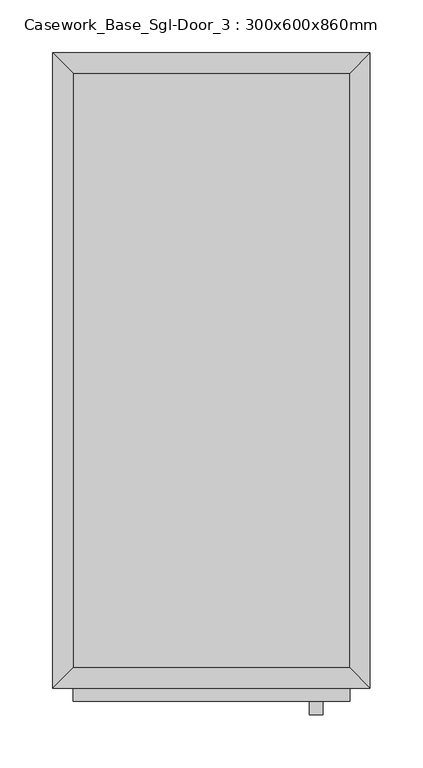
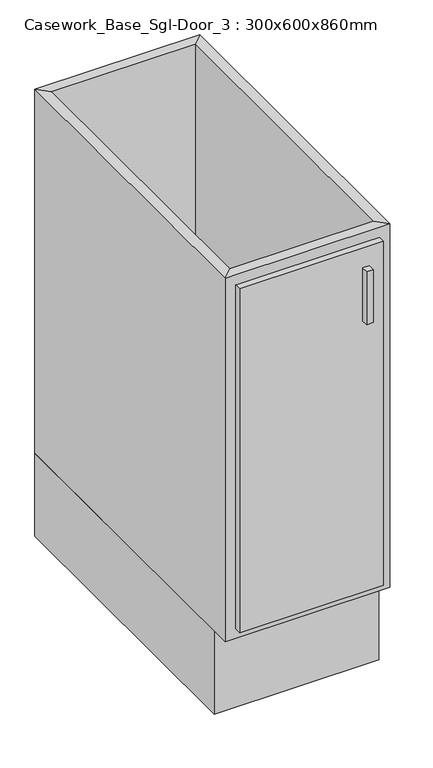
"""IFC4 building model written with IfcOpenShell, lengths in millimetres: furniture geometry, Casework_Base_Sgl-Door_3 : 300x600x860mm."""

import ifcopenshell
import ifcopenshell.guid

model = None  # the IFC model being written
_history = None  # IfcOwnerHistory: only IFC2X3 demands one
_inside = {}  # id of a spatial element -> (the spatial element, [elements in it])
_under = {}  # id of a project, library or spatial element -> (it, [spatial elements below it])
_declared = {}  # id of a project -> (the project, [libraries it declares])
_typed = {}  # id of a type object -> (the type object, [elements of that type])
_made_of = {}  # id of a material, layer set ... -> (it, [elements and type objects made of it])


def new_model(schema):
    """Start an empty IFC model of exactly this schema.

    Asked for "IFC4X3", IfcOpenShell would pick the latest addendum, in which some entities
    have other attributes; the version numbers below select the first issue.
    IFC2X3 requires an IfcOwnerHistory on every rooted entity: one is made here for all.
    """
    global model, _history
    if schema == "IFC4X3":
        model = ifcopenshell.file(schema_version=(4, 3, 0, 0))
    else:
        model = ifcopenshell.file(schema=schema)
    _inside.clear()
    _under.clear()
    _declared.clear()
    _typed.clear()
    _made_of.clear()
    _history = None
    if model.schema == "IFC2X3":
        org = make("IfcOrganization", Name="unknown")
        user = make(
            "IfcPersonAndOrganization",
            ThePerson=make("IfcPerson", FamilyName="unknown"),
            TheOrganization=org,
        )
        app = make(
            "IfcApplication",
            ApplicationDeveloper=org,
            Version="unknown",
            ApplicationFullName="unknown",
            ApplicationIdentifier="unknown",
        )
        _history = make(
            "IfcOwnerHistory",
            OwningUser=user,
            OwningApplication=app,
            ChangeAction="ADDED",
            CreationDate=0,
        )
    return model


def make(cls, **values):
    """One entity of the class cls with the attributes given. An attribute that is None is left unset."""
    return model.create_entity(
        cls, **{name: value for name, value in values.items() if value is not None}
    )


def rooted(cls, **values):
    """An entity with a GlobalId (a new one), such as an element, a storey or a relation."""
    return make(cls, GlobalId=ifcopenshell.guid.new(), OwnerHistory=_history, **values)


def si_unit(unit_type, name, prefix=None):
    """IfcSIUnit, for example si_unit("LENGTHUNIT", "METRE", prefix="MILLI")."""
    return make("IfcSIUnit", UnitType=unit_type, Prefix=prefix, Name=name)


def assignment(units):
    """IfcUnitAssignment: the units of a project."""
    return None if units is None else make("IfcUnitAssignment", Units=units)


def point(xyz):
    """IfcCartesianPoint."""
    return None if xyz is None else make("IfcCartesianPoint", Coordinates=xyz)


def direction(xyz):
    """IfcDirection."""
    return None if xyz is None else make("IfcDirection", DirectionRatios=xyz)


def frame(location, z_axis=None, x_axis=None):
    """IfcAxis2Placement3D, a coordinate frame: its origin and axes. An axis left out is left unset."""
    return make(
        "IfcAxis2Placement3D",
        Location=point(location),
        Axis=direction(z_axis),
        RefDirection=direction(x_axis),
    )


def origin():
    """The frame at (0, 0, 0) with its axes left unset."""
    return frame((0.0, 0.0, 0.0))


def origin_with_axes():
    """The frame at (0, 0, 0) with the z axis (0, 0, 1) and the x axis (1, 0, 0) written out."""
    return frame((0.0, 0.0, 0.0), z_axis=(0.0, 0.0, 1.0), x_axis=(1.0, 0.0, 0.0))


def place(relative_to, where):
    """IfcLocalPlacement: puts the frame where relative to a parent placement (None: the world)."""
    return make(
        "IfcLocalPlacement", PlacementRelTo=relative_to, RelativePlacement=where
    )


def context(
    kind, dimensions, precision=None, world=None, true_north=None, identifier=None
):
    """IfcGeometricRepresentationContext, for example the 3D "Model" context."""
    return make(
        "IfcGeometricRepresentationContext",
        ContextIdentifier=identifier,
        ContextType=kind,
        CoordinateSpaceDimension=dimensions,
        Precision=precision,
        WorldCoordinateSystem=world,
        TrueNorth=true_north,
    )


def project(units=None, contexts=None):
    """IfcProject with its units and contexts."""
    return rooted(
        "IfcProject",
        Name="project",
        RepresentationContexts=contexts,
        UnitsInContext=assignment(units),
    )


def spatial(cls, under=None, at=None, **own):
    """A site, building, storey or space (cls), placed at a placement, below another one or the project."""
    s = rooted(cls, ObjectPlacement=at, **own)
    if under is not None:
        _under.setdefault(under.id(), (under, []))[1].append(s)
    return s


def polyline(points):
    """IfcPolyline through the points."""
    return make("IfcPolyline", Points=[point(p) for p in points])


def outline(outer, holes=None, kind="AREA"):
    """IfcArbitraryClosedProfileDef: a profile drawn as a closed curve; with holes, ...WithVoids."""
    if holes is None:
        return make("IfcArbitraryClosedProfileDef", ProfileType=kind, OuterCurve=outer)
    return make(
        "IfcArbitraryProfileDefWithVoids",
        ProfileType=kind,
        OuterCurve=outer,
        InnerCurves=holes,
    )


def extrude(swept, where, along, depth):
    """IfcExtrudedAreaSolid: the profile swept, set in the frame where, extruded along a direction by depth."""
    return make(
        "IfcExtrudedAreaSolid",
        SweptArea=swept,
        Position=where,
        ExtrudedDirection=direction(along),
        Depth=depth,
    )


def faces_of(points, faces, orient=None, outer=None):
    """IfcFace entities. A face is a list of loops; a loop is a list of indices into points, from 0.

    orient and outer hold one flag for each loop. By default every Orientation is true, the
    first loop of a face is its IfcFaceOuterBound and the others are IfcFaceBound.
    """
    made = []
    for i, loops in enumerate(faces):
        bounds = []
        for j, loop in enumerate(loops):
            is_outer = j == 0 if outer is None else outer[i][j]
            bounds.append(
                make(
                    "IfcFaceOuterBound" if is_outer else "IfcFaceBound",
                    Bound=make("IfcPolyLoop", Polygon=[points[k] for k in loop]),
                    Orientation=True if orient is None else orient[i][j],
                )
            )
        made.append(make("IfcFace", Bounds=bounds))
    return made


def faceted_brep(points, faces, orient=None, outer=None, voids=None):
    """IfcFacetedBrep: a solid bounded by flat faces; with voids (closed shells), ...WithVoids."""
    shared = [point(p) for p in points]
    hull = make("IfcClosedShell", CfsFaces=faces_of(shared, faces, orient, outer))
    if voids is None:
        return make("IfcFacetedBrep", Outer=hull)
    return make(
        "IfcFacetedBrepWithVoids",
        Outer=hull,
        Voids=[
            make(cls, CfsFaces=faces_of(shared, fs, o, b)) for cls, fs, o, b in voids
        ],
    )


def shape(context_of_items, identifier, shape_type, items):
    """IfcShapeRepresentation: the items that make up one representation, for example the "Body"."""
    return make(
        "IfcShapeRepresentation",
        ContextOfItems=context_of_items,
        RepresentationIdentifier=identifier,
        RepresentationType=shape_type,
        Items=items,
    )


def source(mapping_origin, context_of_items, identifier, shape_type, items):
    """IfcRepresentationMap: a shape defined once, which mapped items show again and again."""
    return make(
        "IfcRepresentationMap",
        MappingOrigin=mapping_origin,
        MappedRepresentation=shape(context_of_items, identifier, shape_type, items),
    )


def transform(
    local_origin,
    x_axis=None,
    y_axis=None,
    z_axis=None,
    scale=None,
    scale2=None,
    scale3=None,
    uniform=True,
):
    """IfcCartesianTransformationOperator3D, or its non-uniform kind. x_axis, y_axis, z_axis: its Axis1, 2, 3."""
    if uniform:
        return make(
            "IfcCartesianTransformationOperator3D",
            Axis1=direction(x_axis),
            Axis2=direction(y_axis),
            LocalOrigin=point(local_origin),
            Scale=scale,
            Axis3=direction(z_axis),
        )
    return make(
        "IfcCartesianTransformationOperator3DnonUniform",
        Axis1=direction(x_axis),
        Axis2=direction(y_axis),
        LocalOrigin=point(local_origin),
        Scale=scale,
        Axis3=direction(z_axis),
        Scale2=scale2,
        Scale3=scale3,
    )


def mapped(mapping_source, mapping_target):
    """IfcMappedItem: shows the shape of a source again, moved by a transform."""
    return make(
        "IfcMappedItem", MappingSource=mapping_source, MappingTarget=mapping_target
    )


def made_of(thing, what):
    """Note that an element or type object is made of a material, layer set ...; save() writes the relation."""
    if what is not None:
        _made_of.setdefault(what.id(), (what, []))[1].append(thing)
    return thing


def element(
    cls,
    number,
    at=None,
    inside=None,
    cuts=None,
    type_object=None,
    material=None,
    context=None,
    identifier="Body",
    shape_type=None,
    held_by="IfcProductDefinitionShape",
    body=None,
    shapes=None,
    **own,
):
    """One element of the class cls, such as IfcWall. Its Tag is "e" and its number.

    at: its placement. inside: the storey or other place that contains it. cuts: it is an
    opening in that element (IfcRelVoidsElement). A single representation is given by context,
    identifier, shape_type and body (its items); several are given by shapes. held_by: the class
    of the entity that holds the representations. save() writes the other relations.
    """
    e = rooted(cls, Tag="e%d" % number, ObjectPlacement=at, **own)
    if body is not None:
        shapes = [shape(context, identifier, shape_type, body)]
    if shapes is not None:
        e.Representation = make(held_by, Representations=shapes)
    if inside is not None:
        _inside.setdefault(inside.id(), (inside, []))[1].append(e)
    if cuts is not None:
        rooted(
            "IfcRelVoidsElement", RelatingBuildingElement=cuts, RelatedOpeningElement=e
        )
    if type_object is not None:
        _typed.setdefault(type_object.id(), (type_object, []))[1].append(e)
    return made_of(e, material)


def aggregate(whole, parts):
    """IfcRelAggregates: a whole, such as a stair, and the parts it consists of."""
    return rooted("IfcRelAggregates", RelatingObject=whole, RelatedObjects=parts)


def save(model, path):
    """Write the relations noted so far, then the file.

    IfcRelAggregates (storeys below a building ...), IfcRelContainedInSpatialStructure (elements
    in a storey), IfcRelDefinesByType, IfcRelAssociatesMaterial and IfcRelDeclares: one each for
    every whole, place, type object, material and project.
    """
    for whole, parts in _under.values():
        aggregate(whole, parts)
    for where, things in _inside.values():
        rooted(
            "IfcRelContainedInSpatialStructure",
            RelatedElements=things,
            RelatingStructure=where,
        )
    for kind, things in _typed.values():
        rooted("IfcRelDefinesByType", RelatedObjects=things, RelatingType=kind)
    for what, things in _made_of.values():
        rooted("IfcRelAssociatesMaterial", RelatedObjects=things, RelatingMaterial=what)
    for by, libraries in _declared.values():
        rooted("IfcRelDeclares", RelatingContext=by, RelatedDefinitions=libraries)
    model.write(path)


def casework_base_sgl_door_3_300x600x860mm_ce4f0042(model_context):
    return source(origin(), model_context, "Body", "SolidModel", [
        extrude(outline(polyline([(149.6877049, -19.05), (149.6877049, -580.95), (-112.2122951, -580.95), (-112.2122951, -19.05), (149.6877049, -19.05)])), frame((0.0, 0.0, 160.0), z_axis=(0.0, 0.0, 1.0), x_axis=(1.0, 0.0, 0.0)), (0.0, 0.0, 1.0), 19.05),
        faceted_brep([(149.6877049, -580.95, 860.0), (149.6877049, -580.95, 160.0), (-112.2122951, -580.95, 160.0), (-112.2122951, -580.95, 860.0), (168.7377049, -600.0, 860.0), (-131.2622951, -600.0, 860.0), (168.7377049, -600.0, 160.0), (-131.2622951, -600.0, 160.0), (-112.2122951, -19.05, 160.0), (-112.2122951, -19.05, 860.0), (-131.2622951, 0.0, 860.0), (-131.2622951, 0.0, 160.0), (149.6877049, -19.05, 160.0), (149.6877049, -19.05, 860.0), (168.7377049, 0.0, 860.0), (168.7377049, 0.0, 160.0)], [[[0, 1, 2, 3]], [[4, 0, 3, 5]], [[6, 4, 5, 7]], [[1, 6, 7, 2]], [[3, 2, 8, 9]], [[5, 3, 9, 10]], [[7, 5, 10, 11]], [[2, 7, 11, 8]], [[9, 8, 12, 13]], [[10, 9, 13, 14]], [[11, 10, 14, 15]], [[8, 11, 15, 12]], [[13, 12, 1, 0]], [[14, 13, 0, 4]], [[15, 14, 4, 6]], [[12, 15, 6, 1]]]),
        extrude(outline(polyline([(168.7377049, 0.0), (168.7377049, -565.0), (-131.2622951, -565.0), (-131.2622951, 0.0), (168.7377049, 0.0)])), origin_with_axes(), (0.0, 0.0, 1.0), 160.0),
        extrude(outline(polyline([(124.2877049, -625.4), (111.5877049, -625.4), (111.5877049, -612.7), (124.2877049, -612.7), (124.2877049, -625.4)])), frame((0.0, 0.0, 701.25), z_axis=(0.0, 0.0, 1.0), x_axis=(1.0, 0.0, 0.0)), (0.0, 0.0, 1.0), 101.6),
        extrude(outline(polyline([(149.6877049, -612.7), (-112.2122951, -612.7), (-112.2122951, -600.0), (149.6877049, -600.0), (149.6877049, -612.7)])), frame((0.0, 0.0, 179.05), z_axis=(0.0, 0.0, 1.0), x_axis=(1.0, 0.0, 0.0)), (0.0, 0.0, 1.0), 661.9),
    ])


if __name__ == "__main__":
    model = new_model("IFC4")
    model_context = context("Model", 3, world=origin())
    ifc_project = project(units=[si_unit("LENGTHUNIT", "METRE", prefix="MILLI")], contexts=[model_context])
    site = spatial("IfcSite", under=ifc_project)
    building = spatial("IfcBuilding", under=site)
    placement = place(None, origin())
    casework_base_sgl_door_3_300x600x860mm_shape = casework_base_sgl_door_3_300x600x860mm_ce4f0042(model_context)
    element("IfcFurniture", 1, ObjectType="Casework_Base_Sgl-Door_3 : 300x600x860mm", at=placement, inside=building, context=model_context, shape_type="MappedRepresentation", body=[
        mapped(casework_base_sgl_door_3_300x600x860mm_shape, transform((0.0, 0.0, 0.0), x_axis=(1.0, 0.0, 0.0), y_axis=(0.0, 1.0, 0.0), z_axis=(0.0, 0.0, 1.0))),
    ])
    save(model, "model.ifc")

# Revit data of these elements
# Type "Casework_Base_Sgl-Door_3 : 300x600x860mm"
#   Keynote = "N10"
#   Depth = 600 mm
#   Height = 860 mm
#   Plinth Depth = 35 mm
#   Plinth Height = 160 mm
#   Width = 300 mm
#   Material Cabinet = Cabinets
#   Material Door/Drawer = Cabinets
#   Material Handle = Cabinets - Handles
#   Default Elevation = 0
# Element 1 (IfcFurniture, "Casework_Base_Sgl-Door_3 : 300x600x860mm")
#   Materials on its faces: "Cabinets", "Cabinets - Handles"
# Materials
#   "Cabinets": class "Miscellaneous", colour RGB 249 249 249, transparency 0
#   "Cabinets - Handles": class "Metal", colour RGB 57 57 57, transparency 0
